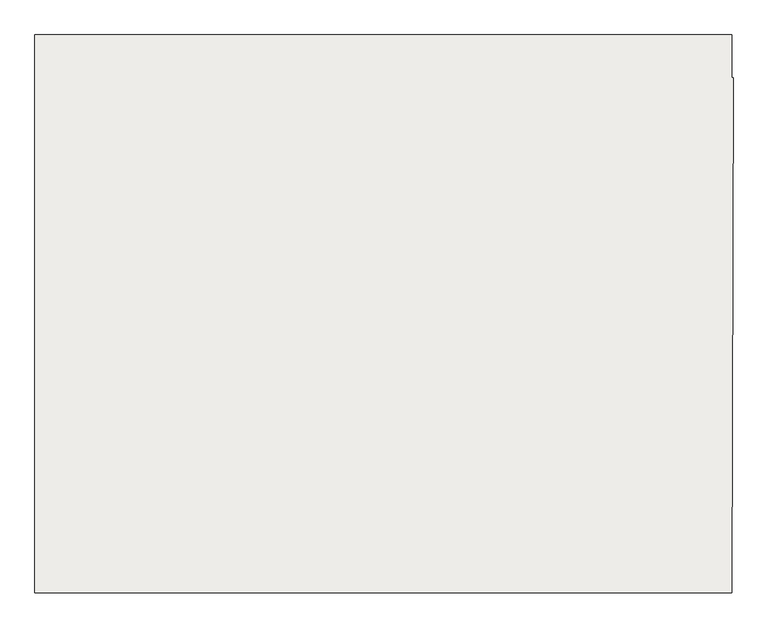
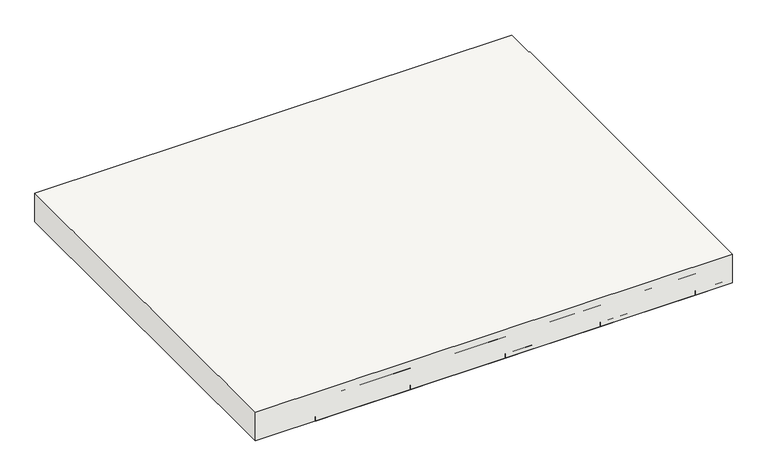
"""IFC4 building model written with IfcOpenShell, lengths in millimetres: slab geometry, Pano 10 (16 cm)."""

from ifc_helpers import new_model, si_unit, origin, origin_with_axes, place, context, project, spatial, polyline, outline, extrude, source, transform, mapped, element, save


def slab_22d407f6(model_context):
    return source(origin(), model_context, "Body", "SweptSolid", [
        extrude(outline(polyline([(-6360.0, 2350.0), (-3850.0, 2350.0), (-3850.0, 2195.0), (-3845.012136, 2195.0), (-3849.514563, 340.0), (-6360.0, 340.0), (-6360.0, 2350.0)])), origin_with_axes(), (0.0, 0.0, 1.0), 160.0),
        extrude(outline(polyline([(-5045.0, 2340.0), (-5405.0, 2340.0), (-5405.0, 2345.0), (-5045.0, 2345.0), (-5045.0, 2340.0)])), origin_with_axes(), (0.0, 0.0, 1.0), 120.0),
        extrude(outline(polyline([(-4045.0, 340.0), (-4405.0, 340.0), (-4405.0, 835.0), (-4045.0, 835.0), (-4045.0, 340.0)])), origin_with_axes(), (0.0, 0.0, 1.0), 120.0),
        extrude(outline(polyline([(-4405.0, 340.0), (-4545.0, 340.0), (-4545.0, 2350.0), (-4405.0, 2350.0), (-4405.0, 340.0)])), origin_with_axes(), (0.0, 0.0, 1.0), 24.0),
        extrude(outline(polyline([(-4045.0, 1840.0), (-4405.0, 1840.0), (-4405.0, 2335.0), (-4045.0, 2335.0), (-4045.0, 1840.0)])), origin_with_axes(), (0.0, 0.0, 1.0), 120.0),
        extrude(outline(polyline([(-5545.0, 840.0), (-5905.0, 840.0), (-5905.0, 1335.0), (-5545.0, 1335.0), (-5545.0, 840.0)])), origin_with_axes(), (0.0, 0.0, 1.0), 120.0),
        extrude(outline(polyline([(-5045.0, 1840.0), (-5405.0, 1840.0), (-5405.0, 2335.0), (-5045.0, 2335.0), (-5045.0, 1840.0)])), origin_with_axes(), (0.0, 0.0, 1.0), 120.0),
        extrude(outline(polyline([(-5545.0, 2340.0), (-5905.0, 2340.0), (-5905.0, 2345.0), (-5545.0, 2345.0), (-5545.0, 2340.0)])), origin_with_axes(), (0.0, 0.0, 1.0), 120.0),
        extrude(outline(polyline([(-5545.0, 1840.0), (-5905.0, 1840.0), (-5905.0, 2335.0), (-5545.0, 2335.0), (-5545.0, 1840.0)])), origin_with_axes(), (0.0, 0.0, 1.0), 120.0),
        extrude(outline(polyline([(-5045.0, 840.0), (-5405.0, 840.0), (-5405.0, 1335.0), (-5045.0, 1335.0), (-5045.0, 840.0)])), origin_with_axes(), (0.0, 0.0, 1.0), 120.0),
        extrude(outline(polyline([(-5905.0, 340.0), (-6045.0, 340.0), (-6045.0, 2350.0), (-5905.0, 2350.0), (-5905.0, 340.0)])), origin_with_axes(), (0.0, 0.0, 1.0), 24.0),
        extrude(outline(polyline([(-4045.0, 2340.0), (-4405.0, 2340.0), (-4405.0, 2345.0), (-4045.0, 2345.0), (-4045.0, 2340.0)])), origin_with_axes(), (0.0, 0.0, 1.0), 120.0),
        extrude(outline(polyline([(-5545.0, 1340.0), (-5905.0, 1340.0), (-5905.0, 1835.0), (-5545.0, 1835.0), (-5545.0, 1340.0)])), origin_with_axes(), (0.0, 0.0, 1.0), 120.0),
        extrude(outline(polyline([(-4045.0, 840.0), (-4405.0, 840.0), (-4405.0, 1335.0), (-4045.0, 1335.0), (-4045.0, 840.0)])), origin_with_axes(), (0.0, 0.0, 1.0), 120.0),
        extrude(outline(polyline([(-5045.0, 1340.0), (-5405.0, 1340.0), (-5405.0, 1835.0), (-5045.0, 1835.0), (-5045.0, 1340.0)])), origin_with_axes(), (0.0, 0.0, 1.0), 120.0),
        extrude(outline(polyline([(-4545.0, 1340.0), (-4905.0, 1340.0), (-4905.0, 1835.0), (-4545.0, 1835.0), (-4545.0, 1340.0)])), origin_with_axes(), (0.0, 0.0, 1.0), 120.0),
        extrude(outline(polyline([(-4905.0, 340.0), (-5045.0, 340.0), (-5045.0, 2350.0), (-4905.0, 2350.0), (-4905.0, 340.0)])), origin_with_axes(), (0.0, 0.0, 1.0), 24.0),
        extrude(outline(polyline([(-4545.0, 340.0), (-4905.0, 340.0), (-4905.0, 835.0), (-4545.0, 835.0), (-4545.0, 340.0)])), origin_with_axes(), (0.0, 0.0, 1.0), 120.0),
        extrude(outline(polyline([(-5405.0, 340.0), (-5545.0, 340.0), (-5545.0, 2350.0), (-5405.0, 2350.0), (-5405.0, 340.0)])), origin_with_axes(), (0.0, 0.0, 1.0), 24.0),
        extrude(outline(polyline([(-4545.0, 840.0), (-4905.0, 840.0), (-4905.0, 1335.0), (-4545.0, 1335.0), (-4545.0, 840.0)])), origin_with_axes(), (0.0, 0.0, 1.0), 120.0),
        extrude(outline(polyline([(-5545.0, 340.0), (-5905.0, 340.0), (-5905.0, 835.0), (-5545.0, 835.0), (-5545.0, 340.0)])), origin_with_axes(), (0.0, 0.0, 1.0), 120.0),
        extrude(outline(polyline([(-4545.0, 2340.0), (-4905.0, 2340.0), (-4905.0, 2345.0), (-4545.0, 2345.0), (-4545.0, 2340.0)])), origin_with_axes(), (0.0, 0.0, 1.0), 120.0),
        extrude(outline(polyline([(-3905.0, 340.0), (-4045.0, 340.0), (-4045.0, 2350.0), (-3905.0, 2350.0), (-3905.0, 340.0)])), origin_with_axes(), (0.0, 0.0, 1.0), 24.0),
        extrude(outline(polyline([(-4545.0, 1840.0), (-4905.0, 1840.0), (-4905.0, 2335.0), (-4545.0, 2335.0), (-4545.0, 1840.0)])), origin_with_axes(), (0.0, 0.0, 1.0), 120.0),
        extrude(outline(polyline([(-5045.0, 340.0), (-5405.0, 340.0), (-5405.0, 835.0), (-5045.0, 835.0), (-5045.0, 340.0)])), origin_with_axes(), (0.0, 0.0, 1.0), 120.0),
        extrude(outline(polyline([(-4045.0, 1340.0), (-4405.0, 1340.0), (-4405.0, 1835.0), (-4045.0, 1835.0), (-4045.0, 1340.0)])), origin_with_axes(), (0.0, 0.0, 1.0), 120.0),
    ])


if __name__ == "__main__":
    model = new_model("IFC4")
    model_context = context("Model", 3, world=origin())
    ifc_project = project(units=[si_unit("LENGTHUNIT", "METRE", prefix="MILLI")], contexts=[model_context])
    site = spatial("IfcSite", under=ifc_project)
    building = spatial("IfcBuilding", under=site)
    placement = place(None, origin())
    slab_shape = slab_22d407f6(model_context)
    element("IfcSlab", 1, ObjectType="Pano 10 (16 cm)", at=placement, inside=building, context=model_context, shape_type="MappedRepresentation", body=[
        mapped(slab_shape, transform((0.0, 0.0, 0.0), x_axis=(1.0, 0.0, 0.0), y_axis=(0.0, 1.0, 0.0), z_axis=(0.0, 0.0, 1.0))),
    ])
    save(model, "model.ifc")

# Revit data of these elements
# Element 1 (IfcSlab, "Pano 10 (16 cm)")
#   Materials on its faces: "Molde de poliestireno", "Concreto armado", "RGB 168-169-158"
# Materials
#   "Molde de poliestireno": class "Não atribuído", colour RGB 255 255 255, transparency 0
#   "Concreto armado": class "Não atribuído", colour RGB 168 169 158, transparency 0
#   "RGB 168-169-158": class "Não atribuído", colour RGB 168 169 158, transparency 0
